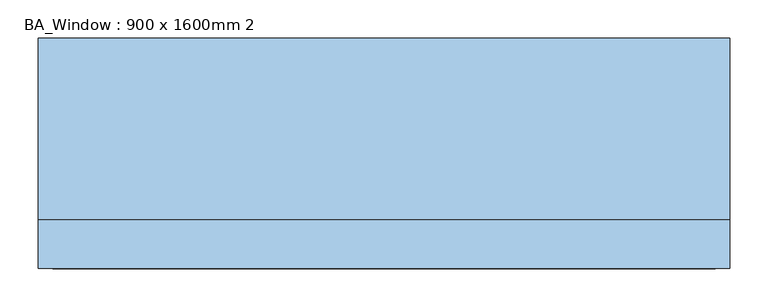
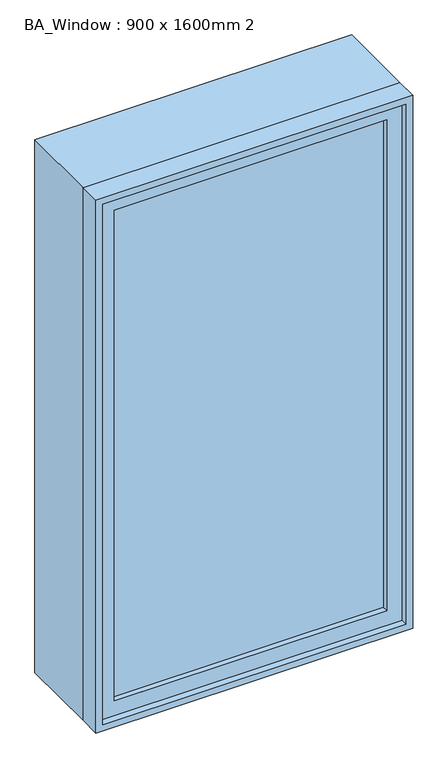
"""IFC4 building model written with IfcOpenShell, lengths in millimetres: window geometry, BA_Window : 900 x 1600mm 2."""

from ifc_helpers import new_model, si_unit, frame, origin, place, context, project, spatial, polyline, outline, extrude, source, transform, mapped, element, save


def ba_window_900_x_1600mm_2_f3ed7943(model_context):
    return source(origin(), model_context, "Body", "SweptSolid", [
        extrude(outline(polyline([(-387.0, -128.0), (-387.0, -116.0), (387.0, -116.0), (387.0, -128.0), (-387.0, -128.0)])), frame((0.0, 0.0, 978.0), z_axis=(0.0, 0.0, 1.0), x_axis=(1.0, 0.0, 0.0)), (0.0, 0.0, 1.0), 1474.0),
        extrude(outline(polyline([(2496.0, -431.0), (934.0, -431.0), (934.0, 431.0), (2496.0, 431.0), (2496.0, -431.0)]), holes=[polyline([(2452.0, -387.0), (2452.0, 387.0), (978.0, 387.0), (978.0, -387.0), (2452.0, -387.0)])]), frame((0.0, -144.0, 0.0), z_axis=(0.0, 1.0, 0.0), x_axis=(0.0, 0.0, 1.0)), (0.0, 0.0, 1.0), 44.0),
        extrude(outline(polyline([(2515.0, -450.0), (915.0, -450.0), (915.0, 450.0), (2515.0, 450.0), (2515.0, -450.0)]), holes=[polyline([(2496.0, -431.0), (2496.0, 431.0), (934.0, 431.0), (934.0, -431.0), (2496.0, -431.0)])]), frame((0.0, -163.0, 0.0), z_axis=(0.0, 1.0, 0.0), x_axis=(0.0, 0.0, 1.0)), (0.0, 0.0, 1.0), 63.0),
        extrude(outline(polyline([(2515.0, -450.0), (915.0, -450.0), (915.0, 450.0), (2515.0, 450.0), (2515.0, -450.0)]), holes=[polyline([(2483.0, -418.0), (2483.0, 418.0), (947.0, 418.0), (947.0, -418.0), (2483.0, -418.0)])]), frame((0.0, -100.0, 0.0), z_axis=(0.0, 1.0, 0.0), x_axis=(0.0, 0.0, 1.0)), (0.0, 0.0, 1.0), 237.0),
    ])


if __name__ == "__main__":
    model = new_model("IFC4")
    model_context = context("Model", 3, world=origin())
    ifc_project = project(units=[si_unit("LENGTHUNIT", "METRE", prefix="MILLI")], contexts=[model_context])
    site = spatial("IfcSite", under=ifc_project)
    building = spatial("IfcBuilding", under=site)
    placement = place(None, origin())
    ba_window_900_x_1600mm_2_shape = ba_window_900_x_1600mm_2_f3ed7943(model_context)
    element("IfcWindow", 1, ObjectType="BA_Window : 900 x 1600mm 2", at=placement, inside=building, context=model_context, shape_type="MappedRepresentation", body=[
        mapped(ba_window_900_x_1600mm_2_shape, transform((0.0, 0.0, 0.0), x_axis=(1.0, 0.0, 0.0), y_axis=(0.0, 1.0, 0.0), z_axis=(0.0, 0.0, 1.0))),
    ])
    save(model, "model.ifc")

# Revit data of these elements
# Type "BA_Window : 900 x 1600mm 2"
#   Type Mark = "40"
#   Construction Type Id = "GSP4R"
#   Analytic Construction = "1/8 in Pilkington single glazing"
#   Visual Light Transmittance = 0.9
#   Thermal Resistance (R) = 0.271106 (m²·K)/W
#   Solar Heat Gain Coefficient = 0.78
#   Heat Transfer Coefficient (U) = 3.6886 W/(m²·K)
#   Height = 1600 mm
#   Default Sill Height = 915 mm
#   Width = 900 mm
#   Window Inset = 19 mm
#   Define Thermal Properties by = 1
#   Frame Exterior Material = Default
#   Frame Interior Material = Default
#   Glass Pane Material = Glass
#   Sash = Default
#   Wall Closure = (empty or 0)
# Element 1 (IfcWindow, "BA_Window : 900 x 1600mm 2")
#   Materials on its faces: "Default", "Glass"
# Materials
#   "Default": class "Generic", colour RGB 255 255 255, transparency 0, Cost = 0
#   "Glass": class "Glass", colour RGB 0 128 192, transparency 0.9, Description = "Soda Lime Glass", Cost = 0
